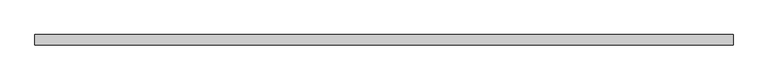
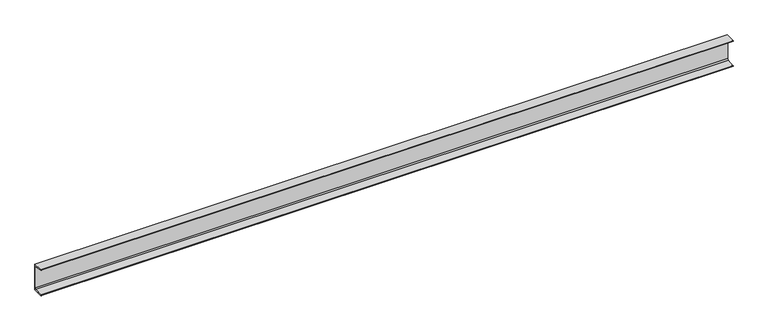
"""IFC4 building model written with IfcOpenShell, lengths in millimetres: beam geometry, C-образный профиль (ГОСТ 8240-89) Балки : [ 22."""

from ifc_helpers import new_model, si_unit, point, frame, frame_2d, origin, place, context, project, spatial, polyline, circle_curve, trimmed, segment, composite_curve, outline, extrude, source, transform, mapped, element, save


def beam_ca0f61b1(model_context):
    return source(origin(), model_context, "Body", "SweptSolid", [
        extrude(outline(composite_curve([segment(polyline([(22.1, 110.0), (22.1, -110.0), (-59.9, -110.0), (-59.9, -108.9686971)]), True, "CONTINUOUS"), segment(trimmed(circle_curve(frame_2d((-55.9, -108.9686971)), 4.0), [point((-59.9, -108.9686971))], [point((-56.3765809, -104.9971897))], False, "CARTESIAN"), True, "CONTINUOUS"), segment(polyline([(-56.3765809, -104.9971897), (7.8914522, -97.2850257)]), True, "CONTINUOUS"), segment(trimmed(circle_curve(frame_2d((6.7, -87.3562574)), 10.0), [point((7.8914522, -97.2850257))], [point((16.7, -87.3562574))], True, "CARTESIAN"), True, "CONTINUOUS"), segment(polyline([(16.7, -87.3562574), (16.7, 87.3562574)]), True, "CONTINUOUS"), segment(trimmed(circle_curve(frame_2d((6.7, 87.3562574)), 10.0), [point((16.7, 87.3562574))], [point((7.8914522, 97.2850257))], True, "CARTESIAN"), True, "CONTINUOUS"), segment(polyline([(7.8914522, 97.2850257), (-56.3765809, 104.9971897)]), True, "CONTINUOUS"), segment(trimmed(circle_curve(frame_2d((-55.9, 108.9686971)), 4.0), [point((-56.3765809, 104.9971897))], [point((-59.9, 108.9686971))], False, "CARTESIAN"), True, "CONTINUOUS"), segment(polyline([(-59.9, 108.9686971), (-59.9, 110.0), (22.1, 110.0)]), True, "CONTINUOUS")], self_intersect=False)), frame((-2805.0, 0.0, 0.0), z_axis=(1.0, 0.0, 0.0), x_axis=(0.0, 1.0, 0.0)), (0.0, 0.0, 1.0), 5610.0),
    ])


if __name__ == "__main__":
    model = new_model("IFC4")
    model_context = context("Model", 3, world=origin())
    ifc_project = project(units=[si_unit("LENGTHUNIT", "METRE", prefix="MILLI")], contexts=[model_context])
    site = spatial("IfcSite", under=ifc_project)
    building = spatial("IfcBuilding", under=site)
    placement = place(None, origin())
    beam_shape = beam_ca0f61b1(model_context)
    element("IfcBeam", 1, ObjectType="C-образный профиль (ГОСТ 8240-89) Балки : [ 22", at=placement, inside=building, context=model_context, shape_type="MappedRepresentation", body=[
        mapped(beam_shape, transform((0.0, 0.0, 0.0), x_axis=(1.0, 0.0, 0.0), y_axis=(0.0, 1.0, 0.0), z_axis=(0.0, 0.0, 1.0))),
    ])
    save(model, "model.ifc")

# Revit data of these elements
# Type "C-образный профиль (ГОСТ 8240-89) Балки : [ 22"
#   tf = 9.5 mm
#   ri = 4 mm
#   ra = 10 mm
#   W = 0.20594
#   Vz = 110 mm
#   Vy = 59.9 mm
#   Vpz = 110 mm
#   Vpy = 22.1 mm
#   Уклон = 0.12
#   Length [instance default] = 1500 mm
#   bf = 82 mm
#   d = 220 mm
#   tw = 5.4 mm
#   A = 0.00267 m²
#   Structural Material [instance default] = Металл - Сталь - 345 МПa
#   Assembly Code = ""
# Element 1 (IfcBeam, "C-образный профиль (ГОСТ 8240-89) Балки : [ 22")
#   Structural Material = C235
#   Materials on its faces: "C235"
# Materials
#   "Металл - Сталь - 345 МПa": class "Металл", colour RGB 247 247 247, transparency 0
#   "C235": class "Не назначено", colour RGB 0 0 0, transparency 0
